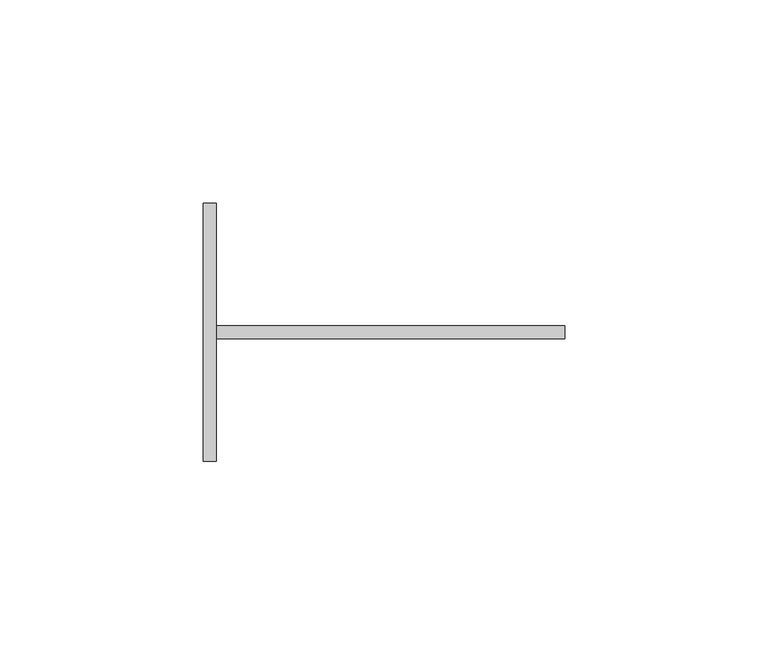
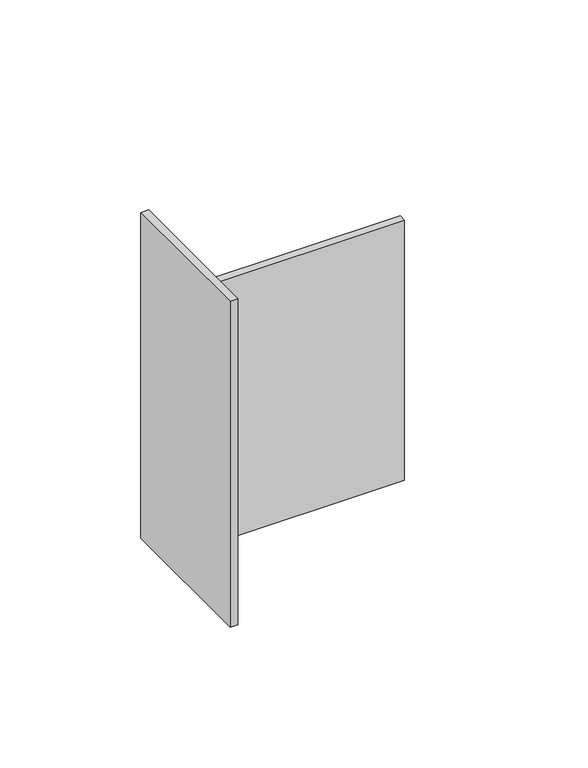
"""IFC4 building model written with IfcOpenShell, lengths in millimetres: proxy geometry, 060523 - W_P_C - Fastenings - Concealed Joist Ties:060523 - W_P_C - Fastenings - Concealed Joist Ties:152592 : 060523 - W_P_C - Fastenings - Concealed Joist Ties:060523 - W_P_C - Fastenings - Concealed Joist Ties:152592."""

from ifc_helpers import new_model, si_unit, frame, origin, place, context, project, spatial, polyline, outline, extrude, source, transform, mapped, element, save


def generic_models_e0af2248(model_context):
    return source(origin(), model_context, "Body", "SweptSolid", [
        extrude(outline(polyline([(-9293.0235758, 742.571923), (-9293.0235758, 679.071923), (-9296.1985758, 679.071923), (-9296.1985758, 742.571923), (-9293.0235758, 742.571923)])), frame((0.0, 0.0, 3169.0018876), z_axis=(0.0, 0.0, 1.0), x_axis=(1.0, 0.0, 0.0)), (0.0, 0.0, 1.0), 141.2875),
        extrude(outline(polyline([(-9207.2985758, 712.409423), (-9207.2985758, 709.234423), (-9293.0235758, 709.234423), (-9293.0235758, 712.409423), (-9207.2985758, 712.409423)])), frame((0.0, 0.0, 3183.2893876), z_axis=(0.0, 0.0, 1.0), x_axis=(1.0, 0.0, 0.0)), (0.0, 0.0, 1.0), 112.7125),
    ])


if __name__ == "__main__":
    model = new_model("IFC4")
    model_context = context("Model", 3, world=origin())
    ifc_project = project(units=[si_unit("LENGTHUNIT", "METRE", prefix="MILLI")], contexts=[model_context])
    site = spatial("IfcSite", under=ifc_project)
    building = spatial("IfcBuilding", under=site)
    placement = place(None, origin())
    generic_models_shape = generic_models_e0af2248(model_context)
    element("IfcBuildingElementProxy", 1, Name="060523 - W_P_C - Fastenings - Concealed Joist Ties:060523 - W_P_C - Fastenings - Concealed Joist Ties:152592 : 060523 - W_P_C - Fastenings - Concealed Joist Ties:060523 - W_P_C - Fastenings - Concealed Joist Ties:152592", ObjectType="060523 - W_P_C - Fastenings - Concealed Joist Ties:060523 - W_P_C - Fastenings - Concealed Joist Ties:152592 : 060523 - W_P_C - Fastenings - Concealed Joist Ties:060523 - W_P_C - Fastenings - Concealed Joist Ties:152592", at=placement, inside=building, context=model_context, shape_type="MappedRepresentation", body=[
        mapped(generic_models_shape, transform((0.0, 0.0, 0.0), x_axis=(1.0, 0.0, 0.0), y_axis=(0.0, 1.0, 0.0), z_axis=(0.0, 0.0, 1.0))),
    ])
    save(model, "model.ifc")

# Revit data of these elements
# Type "060523 - W_P_C - Fastenings - Concealed Joist Ties:060523 - W_P_C - Fastenings - Concealed Joist Ties:152592 : 060523 - W_P_C - Fastenings - Concealed Joist Ties:060523 - W_P_C - Fastenings - Concealed Joist Ties:152592"
#   NameOverride = "060523 - W_P_C - Fastenings - Concealed Joist Ties:060523 - W_P_C - Fastenings - Concealed Joist Ties:152592"
#   ObjectTypeOverride = "060523 - W_P_C - Fastenings - Concealed Joist Ties:060523 - W_P_C - Fastenings - Concealed Joist Ties"
#   Reference = "060523 - W_P_C - Fastenings - Concealed Joist Ties"
#   Category = "Generic Models"
#   Tag = "152592"
# Element 1 (IfcBuildingElementProxy, "060523 - W_P_C - Fastenings - Concealed Joist Ties:060523 - W_P_C - Fastenings - Concealed Joist Ties:152592 : 060523 - W_P_C - Fastenings - Concealed Joist Ties:060523 - W_P_C - Fastenings - Concealed Joist Ties:152592")
#   Materials on its faces: "_BEAM HANGER (SEE STRUCT. DWGS) 6017"
# Materials
#   "_BEAM HANGER (SEE STRUCT. DWGS) 6017": class "Unassigned", colour RGB 191 191 191, transparency 0
